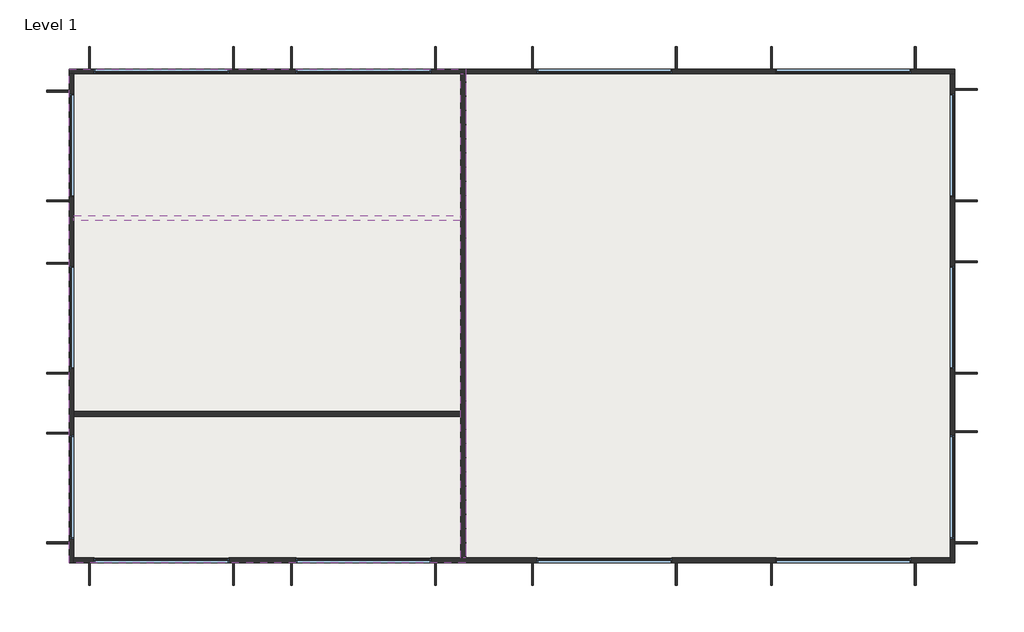
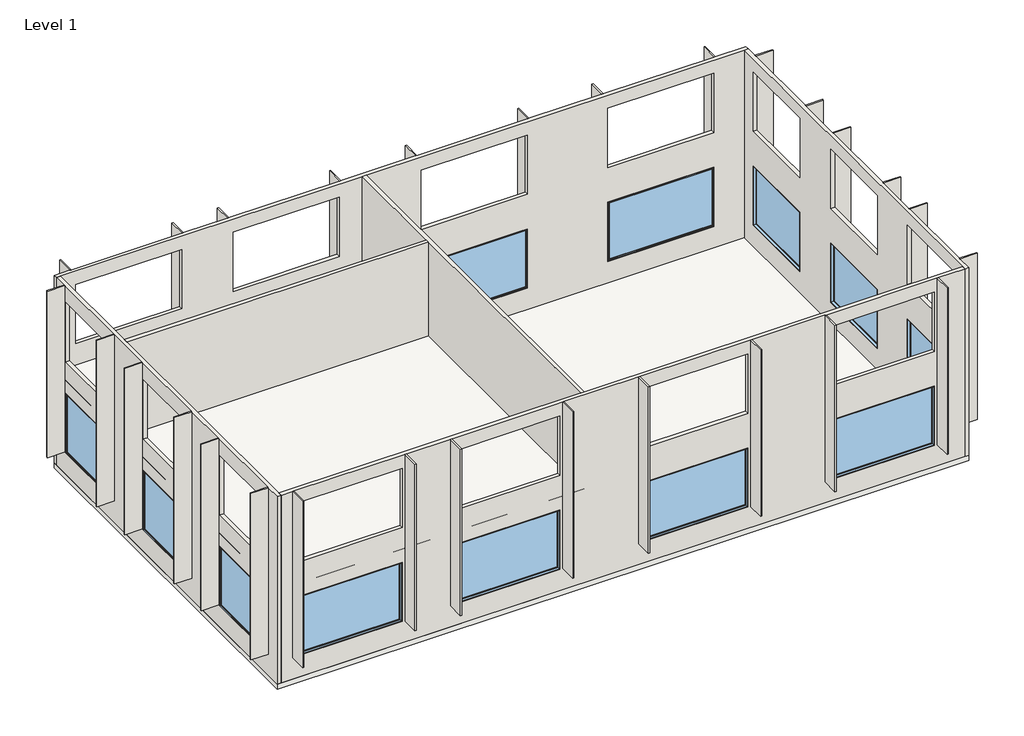
# One storey: 36 walls, 14 windows, 2 slabs.
"""IFC4 building model written with IfcOpenShell, lengths in millimetres."""

import ifcopenshell
import ifcopenshell.guid

model = None  # the IFC model being written
_history = None  # IfcOwnerHistory: only IFC2X3 demands one
_inside = {}  # id of a spatial element -> (the spatial element, [elements in it])
_under = {}  # id of a project, library or spatial element -> (it, [spatial elements below it])
_declared = {}  # id of a project -> (the project, [libraries it declares])
_typed = {}  # id of a type object -> (the type object, [elements of that type])
_made_of = {}  # id of a material, layer set ... -> (it, [elements and type objects made of it])


def new_model(schema):
    """Start an empty IFC model of exactly this schema.

    Asked for "IFC4X3", IfcOpenShell would pick the latest addendum, in which some entities
    have other attributes; the version numbers below select the first issue.
    IFC2X3 requires an IfcOwnerHistory on every rooted entity: one is made here for all.
    """
    global model, _history
    if schema == "IFC4X3":
        model = ifcopenshell.file(schema_version=(4, 3, 0, 0))
    else:
        model = ifcopenshell.file(schema=schema)
    _inside.clear()
    _under.clear()
    _declared.clear()
    _typed.clear()
    _made_of.clear()
    _history = None
    if model.schema == "IFC2X3":
        org = make("IfcOrganization", Name="unknown")
        user = make(
            "IfcPersonAndOrganization",
            ThePerson=make("IfcPerson", FamilyName="unknown"),
            TheOrganization=org,
        )
        app = make(
            "IfcApplication",
            ApplicationDeveloper=org,
            Version="unknown",
            ApplicationFullName="unknown",
            ApplicationIdentifier="unknown",
        )
        _history = make(
            "IfcOwnerHistory",
            OwningUser=user,
            OwningApplication=app,
            ChangeAction="ADDED",
            CreationDate=0,
        )
    return model


def make(cls, **values):
    """One entity of the class cls with the attributes given. An attribute that is None is left unset."""
    return model.create_entity(
        cls, **{name: value for name, value in values.items() if value is not None}
    )


def rooted(cls, **values):
    """An entity with a GlobalId (a new one), such as an element, a storey or a relation."""
    return make(cls, GlobalId=ifcopenshell.guid.new(), OwnerHistory=_history, **values)


def si_unit(unit_type, name, prefix=None):
    """IfcSIUnit, for example si_unit("LENGTHUNIT", "METRE", prefix="MILLI")."""
    return make("IfcSIUnit", UnitType=unit_type, Prefix=prefix, Name=name)


def assignment(units):
    """IfcUnitAssignment: the units of a project."""
    return None if units is None else make("IfcUnitAssignment", Units=units)


def point(xyz):
    """IfcCartesianPoint."""
    return None if xyz is None else make("IfcCartesianPoint", Coordinates=xyz)


def direction(xyz):
    """IfcDirection."""
    return None if xyz is None else make("IfcDirection", DirectionRatios=xyz)


def frame(location, z_axis=None, x_axis=None):
    """IfcAxis2Placement3D, a coordinate frame: its origin and axes. An axis left out is left unset."""
    return make(
        "IfcAxis2Placement3D",
        Location=point(location),
        Axis=direction(z_axis),
        RefDirection=direction(x_axis),
    )


def origin():
    """The frame at (0, 0, 0) with its axes left unset."""
    return frame((0.0, 0.0, 0.0))


def origin_with_axes():
    """The frame at (0, 0, 0) with the z axis (0, 0, 1) and the x axis (1, 0, 0) written out."""
    return frame((0.0, 0.0, 0.0), z_axis=(0.0, 0.0, 1.0), x_axis=(1.0, 0.0, 0.0))


def place(relative_to, where):
    """IfcLocalPlacement: puts the frame where relative to a parent placement (None: the world)."""
    return make(
        "IfcLocalPlacement", PlacementRelTo=relative_to, RelativePlacement=where
    )


def context(
    kind, dimensions, precision=None, world=None, true_north=None, identifier=None
):
    """IfcGeometricRepresentationContext, for example the 3D "Model" context."""
    return make(
        "IfcGeometricRepresentationContext",
        ContextIdentifier=identifier,
        ContextType=kind,
        CoordinateSpaceDimension=dimensions,
        Precision=precision,
        WorldCoordinateSystem=world,
        TrueNorth=true_north,
    )


def project(units=None, contexts=None):
    """IfcProject with its units and contexts."""
    return rooted(
        "IfcProject",
        Name="project",
        RepresentationContexts=contexts,
        UnitsInContext=assignment(units),
    )


def spatial(cls, under=None, at=None, **own):
    """A site, building, storey or space (cls), placed at a placement, below another one or the project."""
    s = rooted(cls, ObjectPlacement=at, **own)
    if under is not None:
        _under.setdefault(under.id(), (under, []))[1].append(s)
    return s


def polyline(points):
    """IfcPolyline through the points."""
    return make("IfcPolyline", Points=[point(p) for p in points])


def outline(outer, holes=None, kind="AREA"):
    """IfcArbitraryClosedProfileDef: a profile drawn as a closed curve; with holes, ...WithVoids."""
    if holes is None:
        return make("IfcArbitraryClosedProfileDef", ProfileType=kind, OuterCurve=outer)
    return make(
        "IfcArbitraryProfileDefWithVoids",
        ProfileType=kind,
        OuterCurve=outer,
        InnerCurves=holes,
    )


def extrude(swept, where, along, depth):
    """IfcExtrudedAreaSolid: the profile swept, set in the frame where, extruded along a direction by depth."""
    return make(
        "IfcExtrudedAreaSolid",
        SweptArea=swept,
        Position=where,
        ExtrudedDirection=direction(along),
        Depth=depth,
    )


def faces_of(points, faces, orient=None, outer=None):
    """IfcFace entities. A face is a list of loops; a loop is a list of indices into points, from 0.

    orient and outer hold one flag for each loop. By default every Orientation is true, the
    first loop of a face is its IfcFaceOuterBound and the others are IfcFaceBound.
    """
    made = []
    for i, loops in enumerate(faces):
        bounds = []
        for j, loop in enumerate(loops):
            is_outer = j == 0 if outer is None else outer[i][j]
            bounds.append(
                make(
                    "IfcFaceOuterBound" if is_outer else "IfcFaceBound",
                    Bound=make("IfcPolyLoop", Polygon=[points[k] for k in loop]),
                    Orientation=True if orient is None else orient[i][j],
                )
            )
        made.append(make("IfcFace", Bounds=bounds))
    return made


def faceted_brep(points, faces, orient=None, outer=None, voids=None):
    """IfcFacetedBrep: a solid bounded by flat faces; with voids (closed shells), ...WithVoids."""
    shared = [point(p) for p in points]
    hull = make("IfcClosedShell", CfsFaces=faces_of(shared, faces, orient, outer))
    if voids is None:
        return make("IfcFacetedBrep", Outer=hull)
    return make(
        "IfcFacetedBrepWithVoids",
        Outer=hull,
        Voids=[
            make(cls, CfsFaces=faces_of(shared, fs, o, b)) for cls, fs, o, b in voids
        ],
    )


def shape(context_of_items, identifier, shape_type, items):
    """IfcShapeRepresentation: the items that make up one representation, for example the "Body"."""
    return make(
        "IfcShapeRepresentation",
        ContextOfItems=context_of_items,
        RepresentationIdentifier=identifier,
        RepresentationType=shape_type,
        Items=items,
    )


def source(mapping_origin, context_of_items, identifier, shape_type, items):
    """IfcRepresentationMap: a shape defined once, which mapped items show again and again."""
    return make(
        "IfcRepresentationMap",
        MappingOrigin=mapping_origin,
        MappedRepresentation=shape(context_of_items, identifier, shape_type, items),
    )


def transform(
    local_origin,
    x_axis=None,
    y_axis=None,
    z_axis=None,
    scale=None,
    scale2=None,
    scale3=None,
    uniform=True,
):
    """IfcCartesianTransformationOperator3D, or its non-uniform kind. x_axis, y_axis, z_axis: its Axis1, 2, 3."""
    if uniform:
        return make(
            "IfcCartesianTransformationOperator3D",
            Axis1=direction(x_axis),
            Axis2=direction(y_axis),
            LocalOrigin=point(local_origin),
            Scale=scale,
            Axis3=direction(z_axis),
        )
    return make(
        "IfcCartesianTransformationOperator3DnonUniform",
        Axis1=direction(x_axis),
        Axis2=direction(y_axis),
        LocalOrigin=point(local_origin),
        Scale=scale,
        Axis3=direction(z_axis),
        Scale2=scale2,
        Scale3=scale3,
    )


def mapped(mapping_source, mapping_target):
    """IfcMappedItem: shows the shape of a source again, moved by a transform."""
    return make(
        "IfcMappedItem", MappingSource=mapping_source, MappingTarget=mapping_target
    )


def made_of(thing, what):
    """Note that an element or type object is made of a material, layer set ...; save() writes the relation."""
    if what is not None:
        _made_of.setdefault(what.id(), (what, []))[1].append(thing)
    return thing


def element(
    cls,
    number,
    at=None,
    inside=None,
    cuts=None,
    type_object=None,
    material=None,
    context=None,
    identifier="Body",
    shape_type=None,
    held_by="IfcProductDefinitionShape",
    body=None,
    shapes=None,
    **own,
):
    """One element of the class cls, such as IfcWall. Its Tag is "e" and its number.

    at: its placement. inside: the storey or other place that contains it. cuts: it is an
    opening in that element (IfcRelVoidsElement). A single representation is given by context,
    identifier, shape_type and body (its items); several are given by shapes. held_by: the class
    of the entity that holds the representations. save() writes the other relations.
    """
    e = rooted(cls, Tag="e%d" % number, ObjectPlacement=at, **own)
    if body is not None:
        shapes = [shape(context, identifier, shape_type, body)]
    if shapes is not None:
        e.Representation = make(held_by, Representations=shapes)
    if inside is not None:
        _inside.setdefault(inside.id(), (inside, []))[1].append(e)
    if cuts is not None:
        rooted(
            "IfcRelVoidsElement", RelatingBuildingElement=cuts, RelatedOpeningElement=e
        )
    if type_object is not None:
        _typed.setdefault(type_object.id(), (type_object, []))[1].append(e)
    return made_of(e, material)


def aggregate(whole, parts):
    """IfcRelAggregates: a whole, such as a stair, and the parts it consists of."""
    return rooted("IfcRelAggregates", RelatingObject=whole, RelatedObjects=parts)


def save(model, path):
    """Write the relations noted so far, then the file.

    IfcRelAggregates (storeys below a building ...), IfcRelContainedInSpatialStructure (elements
    in a storey), IfcRelDefinesByType, IfcRelAssociatesMaterial and IfcRelDeclares: one each for
    every whole, place, type object, material and project.
    """
    for whole, parts in _under.values():
        aggregate(whole, parts)
    for where, things in _inside.values():
        rooted(
            "IfcRelContainedInSpatialStructure",
            RelatedElements=things,
            RelatingStructure=where,
        )
    for kind, things in _typed.values():
        rooted("IfcRelDefinesByType", RelatedObjects=things, RelatingType=kind)
    for what, things in _made_of.values():
        rooted("IfcRelAssociatesMaterial", RelatedObjects=things, RelatingMaterial=what)
    for by, libraries in _declared.values():
        rooted("IfcRelDeclares", RelatingContext=by, RelatedDefinitions=libraries)
    model.write(path)


def m_fixed_2500x_4228mm_fd5e51e7(model_context):
    return source(origin(), model_context, "Body", "SweptSolid", [
        extrude(outline(polyline([(-2050.8, 54.2), (2050.8, 54.2), (2050.8, 42.2), (-2050.8, 42.2), (-2050.8, 54.2)])), frame((0.0, 0.0, 368.0), z_axis=(0.0, 0.0, 1.0), x_axis=(1.0, 0.0, 0.0)), (0.0, 0.0, 1.0), 2374.0),
        extrude(outline(polyline([(2786.0, -2094.8), (324.0, -2094.8), (324.0, 2094.8), (2786.0, 2094.8), (2786.0, -2094.8)]), holes=[polyline([(2742.0, -2050.8), (2742.0, 2050.8), (368.0, 2050.8), (368.0, -2050.8), (2742.0, -2050.8)])]), frame((0.0, 26.2, 0.0), z_axis=(0.0, 1.0, 0.0), x_axis=(0.0, 0.0, 1.0)), (0.0, 0.0, 1.0), 44.0),
        extrude(outline(polyline([(2805.0, -2113.8), (305.0, -2113.8), (305.0, 2113.8), (2805.0, 2113.8), (2805.0, -2113.8)]), holes=[polyline([(2786.0, -2094.8), (2786.0, 2094.8), (324.0, 2094.8), (324.0, -2094.8), (2786.0, -2094.8)])]), frame((0.0, 26.2, 0.0), z_axis=(0.0, 1.0, 0.0), x_axis=(0.0, 0.0, 1.0)), (0.0, 0.0, 1.0), 63.0),
        extrude(outline(polyline([(2805.0, -2113.8), (305.0, -2113.8), (305.0, 2113.8), (2805.0, 2113.8), (2805.0, -2113.8)]), holes=[polyline([(2773.0, -2081.8), (2773.0, 2081.8), (337.0, 2081.8), (337.0, -2081.8), (2773.0, -2081.8)])]), frame((0.0, -63.2, 0.0), z_axis=(0.0, 1.0, 0.0), x_axis=(0.0, 0.0, 1.0)), (0.0, 0.0, 1.0), 89.4),
    ])


def m_fixed_2500x_4228mm_f14c179f(model_context):
    return source(origin(), model_context, "Body", "SweptSolid", [
        extrude(outline(polyline([(-2050.8, -54.2), (-2050.8, -42.2), (2050.8, -42.2), (2050.8, -54.2), (-2050.8, -54.2)])), frame((0.0, 0.0, 368.0), z_axis=(0.0, 0.0, 1.0), x_axis=(1.0, 0.0, 0.0)), (0.0, 0.0, 1.0), 2374.0),
        extrude(outline(polyline([(2786.0, -2094.8), (324.0, -2094.8), (324.0, 2094.8), (2786.0, 2094.8), (2786.0, -2094.8)]), holes=[polyline([(2742.0, -2050.8), (2742.0, 2050.8), (368.0, 2050.8), (368.0, -2050.8), (2742.0, -2050.8)])]), frame((0.0, -70.2, 0.0), z_axis=(0.0, 1.0, 0.0), x_axis=(0.0, 0.0, 1.0)), (0.0, 0.0, 1.0), 44.0),
        extrude(outline(polyline([(2805.0, -2113.8), (305.0, -2113.8), (305.0, 2113.8), (2805.0, 2113.8), (2805.0, -2113.8)]), holes=[polyline([(2786.0, -2094.8), (2786.0, 2094.8), (324.0, 2094.8), (324.0, -2094.8), (2786.0, -2094.8)])]), frame((0.0, -89.2, 0.0), z_axis=(0.0, 1.0, 0.0), x_axis=(0.0, 0.0, 1.0)), (0.0, 0.0, 1.0), 63.0),
        extrude(outline(polyline([(2805.0, -2113.8), (305.0, -2113.8), (305.0, 2113.8), (2805.0, 2113.8), (2805.0, -2113.8)]), holes=[polyline([(2773.0, -2081.8), (2773.0, 2081.8), (337.0, 2081.8), (337.0, -2081.8), (2773.0, -2081.8)])]), frame((0.0, -26.2, 0.0), z_axis=(0.0, 1.0, 0.0), x_axis=(0.0, 0.0, 1.0)), (0.0, 0.0, 1.0), 89.4),
    ])


def m_fixed_2500x_3220mm_df94f4d0(model_context):
    return source(origin(), model_context, "Body", "SweptSolid", [
        extrude(outline(polyline([(-1546.8, 54.2), (1546.8, 54.2), (1546.8, 42.2), (-1546.8, 42.2), (-1546.8, 54.2)])), frame((0.0, 0.0, 368.0), z_axis=(0.0, 0.0, 1.0), x_axis=(1.0, 0.0, 0.0)), (0.0, 0.0, 1.0), 2374.0),
        extrude(outline(polyline([(2786.0, -1590.8), (324.0, -1590.8), (324.0, 1590.8), (2786.0, 1590.8), (2786.0, -1590.8)]), holes=[polyline([(2742.0, -1546.8), (2742.0, 1546.8), (368.0, 1546.8), (368.0, -1546.8), (2742.0, -1546.8)])]), frame((0.0, 26.2, 0.0), z_axis=(0.0, 1.0, 0.0), x_axis=(0.0, 0.0, 1.0)), (0.0, 0.0, 1.0), 44.0),
        extrude(outline(polyline([(2805.0, -1609.8), (305.0, -1609.8), (305.0, 1609.8), (2805.0, 1609.8), (2805.0, -1609.8)]), holes=[polyline([(2786.0, -1590.8), (2786.0, 1590.8), (324.0, 1590.8), (324.0, -1590.8), (2786.0, -1590.8)])]), frame((0.0, 26.2, 0.0), z_axis=(0.0, 1.0, 0.0), x_axis=(0.0, 0.0, 1.0)), (0.0, 0.0, 1.0), 63.0),
        extrude(outline(polyline([(2805.0, -1609.8), (305.0, -1609.8), (305.0, 1609.8), (2805.0, 1609.8), (2805.0, -1609.8)]), holes=[polyline([(2773.0, -1577.8), (2773.0, 1577.8), (337.0, 1577.8), (337.0, -1577.8), (2773.0, -1577.8)])]), frame((0.0, -63.2, 0.0), z_axis=(0.0, 1.0, 0.0), x_axis=(0.0, 0.0, 1.0)), (0.0, 0.0, 1.0), 89.4),
    ])


def m_fixed_2500x_3220mm_8b997f8c(model_context):
    return source(origin(), model_context, "Body", "SweptSolid", [
        extrude(outline(polyline([(-1546.8, -54.2), (-1546.8, -42.2), (1546.8, -42.2), (1546.8, -54.2), (-1546.8, -54.2)])), frame((0.0, 0.0, 368.0), z_axis=(0.0, 0.0, 1.0), x_axis=(1.0, 0.0, 0.0)), (0.0, 0.0, 1.0), 2374.0),
        extrude(outline(polyline([(2786.0, -1590.8), (324.0, -1590.8), (324.0, 1590.8), (2786.0, 1590.8), (2786.0, -1590.8)]), holes=[polyline([(2742.0, -1546.8), (2742.0, 1546.8), (368.0, 1546.8), (368.0, -1546.8), (2742.0, -1546.8)])]), frame((0.0, -70.2, 0.0), z_axis=(0.0, 1.0, 0.0), x_axis=(0.0, 0.0, 1.0)), (0.0, 0.0, 1.0), 44.0),
        extrude(outline(polyline([(2805.0, -1609.8), (305.0, -1609.8), (305.0, 1609.8), (2805.0, 1609.8), (2805.0, -1609.8)]), holes=[polyline([(2786.0, -1590.8), (2786.0, 1590.8), (324.0, 1590.8), (324.0, -1590.8), (2786.0, -1590.8)])]), frame((0.0, -89.2, 0.0), z_axis=(0.0, 1.0, 0.0), x_axis=(0.0, 0.0, 1.0)), (0.0, 0.0, 1.0), 63.0),
        extrude(outline(polyline([(2805.0, -1609.8), (305.0, -1609.8), (305.0, 1609.8), (2805.0, 1609.8), (2805.0, -1609.8)]), holes=[polyline([(2773.0, -1577.8), (2773.0, 1577.8), (337.0, 1577.8), (337.0, -1577.8), (2773.0, -1577.8)])]), frame((0.0, -26.2, 0.0), z_axis=(0.0, 1.0, 0.0), x_axis=(0.0, 0.0, 1.0)), (0.0, 0.0, 1.0), 89.4),
    ])


model = new_model("IFC4")

# Units and contexts
model_context = context("Model", 3, world=origin())
ifc_project = project(units=[si_unit("LENGTHUNIT", "METRE", prefix="MILLI")], contexts=[model_context])

# Site, building, storey
site = spatial("IfcSite", under=ifc_project)
building = spatial("IfcBuilding", under=site)
storey = spatial("IfcBuildingStorey", under=building, Name="Level 1", Elevation=0.0)

# Slabs
placement = place(None, origin())
element("IfcSlab", 1, ObjectType="160mm Concrete With 50mm Metal Deck", at=placement, inside=storey, context=model_context, shape_type="Brep", body=[
    faceted_brep([(29068.464681, 11296.9802217, -210.0), (29068.464681, -4095.4197783, -210.0), (1484.064681, -4095.4197783, -210.0), (1484.064681, 11296.9802217, -210.0), (29068.464681, 11296.9802217, 0.0), (1484.064681, 11296.9802217, 0.0), (1484.064681, -4095.4197783, 0.0), (28916.064681, -4095.4197783, 0.0), (29068.464681, -4095.4197783, 0.0), (29068.464681, 11144.5802217, 0.0)], [[[0, 1, 2, 3]], [[4, 5, 6, 7, 8, 9]], [[1, 0, 4, 9, 8]], [[2, 1, 8, 7, 6]], [[3, 2, 6, 5]], [[0, 3, 5, 4]]]),
])
element("IfcSlab", 2, ObjectType="160mm Concrete With 50mm Metal Deck", at=placement, inside=storey, context=model_context, shape_type="SweptSolid", body=[
    extrude(outline(polyline([(13828.464681, 11296.9802217), (13828.464681, -4095.4197783), (1484.064681, -4095.4197783), (1484.064681, 11296.9802217), (13828.464681, 11296.9802217)])), frame((0.0, 0.0, 3752.4), z_axis=(0.0, 0.0, 1.0), x_axis=(1.0, 0.0, 0.0)), (0.0, 0.0, 1.0), 210.0),
])

# Walls
element("IfcWall", 3, ObjectType="Generic - 152.4mm", at=placement, inside=storey, context=model_context, shape_type="Brep", body=[
    faceted_brep([(1484.064681, 11144.5802217, 0.0), (1636.464681, 11144.5802217, 0.0), (13676.064681, 11144.5802217, 0.0), (13828.464681, 11144.5802217, 0.0), (28916.064681, 11144.5802217, 0.0), (29068.464681, 11144.5802217, 0.0), (29068.464681, 11144.5802217, 7924.8), (28916.064681, 11144.5802217, 7924.8), (13828.464681, 11144.5802217, 7924.8), (13676.064681, 11144.5802217, 7924.8), (1636.464681, 11144.5802217, 7924.8), (1484.064681, 11144.5802217, 7924.8), (6474.064681, 11144.5802217, 902.4), (2246.464681, 11144.5802217, 902.4), (2246.464681, 11144.5802217, 3402.4), (6474.064681, 11144.5802217, 3402.4), (12766.064681, 11144.5802217, 902.4), (8538.464681, 11144.5802217, 902.4), (8538.464681, 11144.5802217, 3402.4), (12766.064681, 11144.5802217, 3402.4), (20266.064681, 11144.5802217, 902.4), (16038.464681, 11144.5802217, 902.4), (16038.464681, 11144.5802217, 3402.4), (20266.064681, 11144.5802217, 3402.4), (27706.064681, 11144.5802217, 902.4), (23478.464681, 11144.5802217, 902.4), (23478.464681, 11144.5802217, 3402.4), (27706.064681, 11144.5802217, 3402.4), (27706.064681, 11144.5802217, 4862.4), (23478.464681, 11144.5802217, 4862.4), (23478.464681, 11144.5802217, 7362.4), (27706.064681, 11144.5802217, 7362.4), (20266.064681, 11144.5802217, 4862.4), (16038.464681, 11144.5802217, 4862.4), (16038.464681, 11144.5802217, 7362.4), (20266.064681, 11144.5802217, 7362.4), (12766.064681, 11144.5802217, 4862.4), (8538.464681, 11144.5802217, 4862.4), (8538.464681, 11144.5802217, 7362.4), (12766.064681, 11144.5802217, 7362.4), (6474.064681, 11144.5802217, 4862.4), (2246.464681, 11144.5802217, 4862.4), (2246.464681, 11144.5802217, 7362.4), (6474.064681, 11144.5802217, 7362.4), (1484.064681, 11296.9802217, 0.0), (1484.064681, 11296.9802217, 7924.8), (2096.464681, 11296.9802217, 7924.8), (2146.464681, 11296.9802217, 7924.8), (6574.064681, 11296.9802217, 7924.8), (6624.064681, 11296.9802217, 7924.8), (8388.464681, 11296.9802217, 7924.8), (8438.464681, 11296.9802217, 7924.8), (12866.064681, 11296.9802217, 7924.8), (12916.064681, 11296.9802217, 7924.8), (15888.464681, 11296.9802217, 7924.8), (15938.464681, 11296.9802217, 7924.8), (20366.064681, 11296.9802217, 7924.8), (20416.064681, 11296.9802217, 7924.8), (23328.464681, 11296.9802217, 7924.8), (23378.464681, 11296.9802217, 7924.8), (27806.064681, 11296.9802217, 7924.8), (27856.064681, 11296.9802217, 7924.8), (29068.464681, 11296.9802217, 7924.8), (29068.464681, 11296.9802217, 0.0), (6474.064681, 11296.9802217, 902.4), (6474.064681, 11296.9802217, 3402.4), (2246.464681, 11296.9802217, 3402.4), (2246.464681, 11296.9802217, 902.4), (12766.064681, 11296.9802217, 902.4), (12766.064681, 11296.9802217, 3402.4), (8538.464681, 11296.9802217, 3402.4), (8538.464681, 11296.9802217, 902.4), (20266.064681, 11296.9802217, 902.4), (20266.064681, 11296.9802217, 3402.4), (16038.464681, 11296.9802217, 3402.4), (16038.464681, 11296.9802217, 902.4), (27706.064681, 11296.9802217, 902.4), (27706.064681, 11296.9802217, 3402.4), (23478.464681, 11296.9802217, 3402.4), (23478.464681, 11296.9802217, 902.4), (27706.064681, 11296.9802217, 4862.4), (27706.064681, 11296.9802217, 7362.4), (23478.464681, 11296.9802217, 7362.4), (23478.464681, 11296.9802217, 4862.4), (20266.064681, 11296.9802217, 4862.4), (20266.064681, 11296.9802217, 7362.4), (16038.464681, 11296.9802217, 7362.4), (16038.464681, 11296.9802217, 4862.4), (12766.064681, 11296.9802217, 4862.4), (12766.064681, 11296.9802217, 7362.4), (8538.464681, 11296.9802217, 7362.4), (8538.464681, 11296.9802217, 4862.4), (6474.064681, 11296.9802217, 4862.4), (6474.064681, 11296.9802217, 7362.4), (2246.464681, 11296.9802217, 7362.4), (2246.464681, 11296.9802217, 4862.4)], [[[0, 1, 2, 3, 4, 5, 6, 7, 8, 9, 10, 11], [12, 13, 14, 15], [16, 17, 18, 19], [20, 21, 22, 23], [24, 25, 26, 27], [28, 29, 30, 31], [32, 33, 34, 35], [36, 37, 38, 39], [40, 41, 42, 43]], [[44, 45, 46, 47, 48, 49, 50, 51, 52, 53, 54, 55, 56, 57, 58, 59, 60, 61, 62, 63], [64, 65, 66, 67], [68, 69, 70, 71], [72, 73, 74, 75], [76, 77, 78, 79], [80, 81, 82, 83], [84, 85, 86, 87], [88, 89, 90, 91], [92, 93, 94, 95]], [[5, 4, 3, 2, 1, 0, 44, 63]], [[11, 10, 9, 8, 7, 6, 62, 61, 60, 59, 58, 57, 56, 55, 54, 53, 52, 51, 50, 49, 48, 47, 46, 45]], [[6, 5, 63, 62]], [[0, 11, 45, 44]], [[65, 64, 12, 15]], [[66, 65, 15, 14]], [[67, 66, 14, 13]], [[64, 67, 13, 12]], [[69, 68, 16, 19]], [[70, 69, 19, 18]], [[71, 70, 18, 17]], [[68, 71, 17, 16]], [[73, 72, 20, 23]], [[74, 73, 23, 22]], [[75, 74, 22, 21]], [[72, 75, 21, 20]], [[77, 76, 24, 27]], [[78, 77, 27, 26]], [[79, 78, 26, 25]], [[76, 79, 25, 24]], [[81, 80, 28, 31]], [[82, 81, 31, 30]], [[83, 82, 30, 29]], [[80, 83, 29, 28]], [[85, 84, 32, 35]], [[86, 85, 35, 34]], [[87, 86, 34, 33]], [[84, 87, 33, 32]], [[89, 88, 36, 39]], [[90, 89, 39, 38]], [[91, 90, 38, 37]], [[88, 91, 37, 36]], [[93, 92, 40, 43]], [[94, 93, 43, 42]], [[95, 94, 42, 41]], [[92, 95, 41, 40]]]),
])
element("IfcWall", 4, ObjectType="Generic - 152.4mm", at=placement, inside=storey, context=model_context, shape_type="Brep", body=[
    faceted_brep([(28916.064681, 11144.5802217, 0.0), (28916.064681, -3943.0197783, 0.0), (28916.064681, -4095.4197783, 0.0), (28916.064681, -4095.4197783, 7924.8), (28916.064681, -3943.0197783, 7924.8), (28916.064681, 11144.5802217, 7924.8), (28916.064681, -3343.0197783, 902.4), (28916.064681, -123.4197783, 902.4), (28916.064681, -123.4197783, 3402.4), (28916.064681, -3343.0197783, 3402.4), (28916.064681, 1942.9802217, 902.4), (28916.064681, 5162.5802217, 902.4), (28916.064681, 5162.5802217, 3402.4), (28916.064681, 1942.9802217, 3402.4), (28916.064681, 7310.9802217, 902.4), (28916.064681, 10530.5802217, 902.4), (28916.064681, 10530.5802217, 3402.4), (28916.064681, 7310.9802217, 3402.4), (28916.064681, -3343.0197783, 4864.8), (28916.064681, -123.4197783, 4864.8), (28916.064681, -123.4197783, 7364.8), (28916.064681, -3343.0197783, 7364.8), (28916.064681, 1942.9802217, 4864.8), (28916.064681, 5162.5802217, 4864.8), (28916.064681, 5162.5802217, 7364.8), (28916.064681, 1942.9802217, 7364.8), (28916.064681, 7310.9802217, 4864.8), (28916.064681, 10530.5802217, 4864.8), (28916.064681, 10530.5802217, 7364.8), (28916.064681, 7310.9802217, 7364.8), (29068.464681, 11144.5802217, 0.0), (29068.464681, 11144.5802217, 7924.8), (29068.464681, 10680.5802217, 7924.8), (29068.464681, 10630.5802217, 7924.8), (29068.464681, 7210.9802217, 7924.8), (29068.464681, 7160.9802217, 7924.8), (29068.464681, 5312.5802217, 7924.8), (29068.464681, 5262.5802217, 7924.8), (29068.464681, 1842.9802217, 7924.8), (29068.464681, 1792.9802217, 7924.8), (29068.464681, 26.5802217, 7924.8), (29068.464681, -23.4197783, 7924.8), (29068.464681, -3443.0197783, 7924.8), (29068.464681, -3493.0197783, 7924.8), (29068.464681, -4095.4197783, 7924.8), (29068.464681, -4095.4197783, 0.0), (29068.464681, -3343.0197783, 902.4), (29068.464681, -3343.0197783, 3402.4), (29068.464681, -123.4197783, 3402.4), (29068.464681, -123.4197783, 902.4), (29068.464681, 1942.9802217, 902.4), (29068.464681, 1942.9802217, 3402.4), (29068.464681, 5162.5802217, 3402.4), (29068.464681, 5162.5802217, 902.4), (29068.464681, 7310.9802217, 902.4), (29068.464681, 7310.9802217, 3402.4), (29068.464681, 10530.5802217, 3402.4), (29068.464681, 10530.5802217, 902.4), (29068.464681, -3343.0197783, 4864.8), (29068.464681, -3343.0197783, 7364.8), (29068.464681, -123.4197783, 7364.8), (29068.464681, -123.4197783, 4864.8), (29068.464681, 1942.9802217, 4864.8), (29068.464681, 1942.9802217, 7364.8), (29068.464681, 5162.5802217, 7364.8), (29068.464681, 5162.5802217, 4864.8), (29068.464681, 7310.9802217, 4864.8), (29068.464681, 7310.9802217, 7364.8), (29068.464681, 10530.5802217, 7364.8), (29068.464681, 10530.5802217, 4864.8)], [[[0, 1, 2, 3, 4, 5], [6, 7, 8, 9], [10, 11, 12, 13], [14, 15, 16, 17], [18, 19, 20, 21], [22, 23, 24, 25], [26, 27, 28, 29]], [[30, 31, 32, 33, 34, 35, 36, 37, 38, 39, 40, 41, 42, 43, 44, 45], [46, 47, 48, 49], [50, 51, 52, 53], [54, 55, 56, 57], [58, 59, 60, 61], [62, 63, 64, 65], [66, 67, 68, 69]], [[2, 1, 0, 30, 45]], [[5, 4, 3, 44, 43, 42, 41, 40, 39, 38, 37, 36, 35, 34, 33, 32, 31]], [[0, 5, 31, 30]], [[47, 46, 6, 9]], [[48, 47, 9, 8]], [[49, 48, 8, 7]], [[46, 49, 7, 6]], [[51, 50, 10, 13]], [[52, 51, 13, 12]], [[53, 52, 12, 11]], [[50, 53, 11, 10]], [[55, 54, 14, 17]], [[56, 55, 17, 16]], [[57, 56, 16, 15]], [[54, 57, 15, 14]], [[3, 2, 45, 44]], [[59, 58, 18, 21]], [[60, 59, 21, 20]], [[61, 60, 20, 19]], [[58, 61, 19, 18]], [[63, 62, 22, 25]], [[64, 63, 25, 24]], [[65, 64, 24, 23]], [[62, 65, 23, 22]], [[67, 66, 26, 29]], [[68, 67, 29, 28]], [[69, 68, 28, 27]], [[66, 69, 27, 26]]]),
])
element("IfcWall", 5, ObjectType="Generic - 152.4mm", at=placement, inside=storey, context=model_context, shape_type="Brep", body=[
    faceted_brep([(28916.064681, -3943.0197783, 0.0), (13828.464681, -3943.0197783, 0.0), (13676.064681, -3943.0197783, 0.0), (1636.464681, -3943.0197783, 0.0), (1636.464681, -3943.0197783, 7924.8), (13676.064681, -3943.0197783, 7924.8), (13828.464681, -3943.0197783, 7924.8), (28916.064681, -3943.0197783, 7924.8), (27706.064681, -3943.0197783, 902.4), (27706.064681, -3943.0197783, 3402.4), (23478.464681, -3943.0197783, 3402.4), (23478.464681, -3943.0197783, 902.4), (20266.064681, -3943.0197783, 902.4), (20266.064681, -3943.0197783, 3402.4), (16038.464681, -3943.0197783, 3402.4), (16038.464681, -3943.0197783, 902.4), (12766.064681, -3943.0197783, 902.4), (12766.064681, -3943.0197783, 3402.4), (8538.464681, -3943.0197783, 3402.4), (8538.464681, -3943.0197783, 902.4), (6474.064681, -3943.0197783, 902.4), (6474.064681, -3943.0197783, 3402.4), (2246.464681, -3943.0197783, 3402.4), (2246.464681, -3943.0197783, 902.4), (27706.064681, -3943.0197783, 4862.4), (27706.064681, -3943.0197783, 7362.4), (23478.464681, -3943.0197783, 7362.4), (23478.464681, -3943.0197783, 4862.4), (20266.064681, -3943.0197783, 4862.4), (20266.064681, -3943.0197783, 7362.4), (16038.464681, -3943.0197783, 7362.4), (16038.464681, -3943.0197783, 4862.4), (12766.064681, -3943.0197783, 4862.4), (12766.064681, -3943.0197783, 7362.4), (8538.464681, -3943.0197783, 7362.4), (8538.464681, -3943.0197783, 4862.4), (6474.064681, -3943.0197783, 4862.4), (6474.064681, -3943.0197783, 7362.4), (2246.464681, -3943.0197783, 7362.4), (2246.464681, -3943.0197783, 4862.4), (28916.064681, -4095.4197783, 0.0), (28916.064681, -4095.4197783, 7924.8), (27856.064681, -4095.4197783, 7924.8), (27806.064681, -4095.4197783, 7924.8), (23378.464681, -4095.4197783, 7924.8), (23328.464681, -4095.4197783, 7924.8), (20416.064681, -4095.4197783, 7924.8), (20366.064681, -4095.4197783, 7924.8), (15938.464681, -4095.4197783, 7924.8), (15888.464681, -4095.4197783, 7924.8), (12916.064681, -4095.4197783, 7924.8), (12866.064681, -4095.4197783, 7924.8), (8438.464681, -4095.4197783, 7924.8), (8388.464681, -4095.4197783, 7924.8), (6624.064681, -4095.4197783, 7924.8), (6574.064681, -4095.4197783, 7924.8), (2146.464681, -4095.4197783, 7924.8), (2096.464681, -4095.4197783, 7924.8), (1636.464681, -4095.4197783, 7924.8), (1636.464681, -4095.4197783, 0.0), (27706.064681, -4095.4197783, 902.4), (23478.464681, -4095.4197783, 902.4), (23478.464681, -4095.4197783, 3402.4), (27706.064681, -4095.4197783, 3402.4), (20266.064681, -4095.4197783, 902.4), (16038.464681, -4095.4197783, 902.4), (16038.464681, -4095.4197783, 3402.4), (20266.064681, -4095.4197783, 3402.4), (12766.064681, -4095.4197783, 902.4), (8538.464681, -4095.4197783, 902.4), (8538.464681, -4095.4197783, 3402.4), (12766.064681, -4095.4197783, 3402.4), (6474.064681, -4095.4197783, 902.4), (2246.464681, -4095.4197783, 902.4), (2246.464681, -4095.4197783, 3402.4), (6474.064681, -4095.4197783, 3402.4), (27706.064681, -4095.4197783, 4862.4), (23478.464681, -4095.4197783, 4862.4), (23478.464681, -4095.4197783, 7362.4), (27706.064681, -4095.4197783, 7362.4), (20266.064681, -4095.4197783, 4862.4), (16038.464681, -4095.4197783, 4862.4), (16038.464681, -4095.4197783, 7362.4), (20266.064681, -4095.4197783, 7362.4), (12766.064681, -4095.4197783, 4862.4), (8538.464681, -4095.4197783, 4862.4), (8538.464681, -4095.4197783, 7362.4), (12766.064681, -4095.4197783, 7362.4), (6474.064681, -4095.4197783, 4862.4), (2246.464681, -4095.4197783, 4862.4), (2246.464681, -4095.4197783, 7362.4), (6474.064681, -4095.4197783, 7362.4)], [[[0, 1, 2, 3, 4, 5, 6, 7], [8, 9, 10, 11], [12, 13, 14, 15], [16, 17, 18, 19], [20, 21, 22, 23], [24, 25, 26, 27], [28, 29, 30, 31], [32, 33, 34, 35], [36, 37, 38, 39]], [[40, 41, 42, 43, 44, 45, 46, 47, 48, 49, 50, 51, 52, 53, 54, 55, 56, 57, 58, 59], [60, 61, 62, 63], [64, 65, 66, 67], [68, 69, 70, 71], [72, 73, 74, 75], [76, 77, 78, 79], [80, 81, 82, 83], [84, 85, 86, 87], [88, 89, 90, 91]], [[3, 2, 1, 0, 40, 59]], [[7, 6, 5, 4, 58, 57, 56, 55, 54, 53, 52, 51, 50, 49, 48, 47, 46, 45, 44, 43, 42, 41]], [[9, 8, 60, 63]], [[10, 9, 63, 62]], [[11, 10, 62, 61]], [[8, 11, 61, 60]], [[13, 12, 64, 67]], [[14, 13, 67, 66]], [[15, 14, 66, 65]], [[12, 15, 65, 64]], [[17, 16, 68, 71]], [[18, 17, 71, 70]], [[19, 18, 70, 69]], [[16, 19, 69, 68]], [[21, 20, 72, 75]], [[22, 21, 75, 74]], [[23, 22, 74, 73]], [[20, 23, 73, 72]], [[0, 7, 41, 40]], [[4, 3, 59, 58]], [[25, 24, 76, 79]], [[26, 25, 79, 78]], [[27, 26, 78, 77]], [[24, 27, 77, 76]], [[29, 28, 80, 83]], [[30, 29, 83, 82]], [[31, 30, 82, 81]], [[28, 31, 81, 80]], [[33, 32, 84, 87]], [[34, 33, 87, 86]], [[35, 34, 86, 85]], [[32, 35, 85, 84]], [[37, 36, 88, 91]], [[38, 37, 91, 90]], [[39, 38, 90, 89]], [[36, 39, 89, 88]]]),
])
element("IfcWall", 6, ObjectType="Generic - 152.4mm", at=placement, inside=storey, context=model_context, shape_type="Brep", body=[
    faceted_brep([(1636.464681, -4095.4197783, 0.0), (1636.464681, -3943.0197783, 0.0), (1636.464681, 476.5802217, 0.0), (1636.464681, 628.9802217, 0.0), (1636.464681, 11144.5802217, 0.0), (1636.464681, 11144.5802217, 7924.8), (1636.464681, 6724.9802217, 7924.8), (1636.464681, 6572.5802217, 7924.8), (1636.464681, -3943.0197783, 7924.8), (1636.464681, -4095.4197783, 7924.8), (1636.464681, 7310.9802217, 4734.5029682), (1636.464681, 7310.9802217, 7234.5029682), (1636.464681, 10530.5802217, 7234.5029682), (1636.464681, 10530.5802217, 4734.5029682), (1636.464681, 1942.9802217, 4734.5029682), (1636.464681, 1942.9802217, 7234.5029682), (1636.464681, 5162.5802217, 7234.5029682), (1636.464681, 5162.5802217, 4734.5029682), (1636.464681, -3343.0197783, 4734.5029682), (1636.464681, -3343.0197783, 7234.5029682), (1636.464681, -123.4197783, 7234.5029682), (1636.464681, -123.4197783, 4734.5029682), (1636.464681, -3343.0197783, 902.4), (1636.464681, -3343.0197783, 3402.4), (1636.464681, -123.4197783, 3402.4), (1636.464681, -123.4197783, 902.4), (1636.464681, 7310.9802217, 902.4), (1636.464681, 7310.9802217, 3402.4), (1636.464681, 10530.5802217, 3402.4), (1636.464681, 10530.5802217, 902.4), (1636.464681, 1942.9802217, 902.4), (1636.464681, 1942.9802217, 3402.4), (1636.464681, 5162.5802217, 3402.4), (1636.464681, 5162.5802217, 902.4), (1484.064681, -4095.4197783, 0.0), (1484.064681, -4095.4197783, 7924.8), (1484.064681, -3493.0197783, 7924.8), (1484.064681, -3443.0197783, 7924.8), (1484.064681, -73.4197783, 7924.8), (1484.064681, -23.4197783, 7924.8), (1484.064681, 1792.9802217, 7924.8), (1484.064681, 1842.9802217, 7924.8), (1484.064681, 5212.5802217, 7924.8), (1484.064681, 5262.5802217, 7924.8), (1484.064681, 7160.9802217, 7924.8), (1484.064681, 7210.9802217, 7924.8), (1484.064681, 10580.5802217, 7924.8), (1484.064681, 10630.5802217, 7924.8), (1484.064681, 11144.5802217, 7924.8), (1484.064681, 11144.5802217, 0.0), (1484.064681, 7310.9802217, 4734.5029682), (1484.064681, 10530.5802217, 4734.5029682), (1484.064681, 10530.5802217, 7234.5029682), (1484.064681, 7310.9802217, 7234.5029682), (1484.064681, 1942.9802217, 4734.5029682), (1484.064681, 5162.5802217, 4734.5029682), (1484.064681, 5162.5802217, 7234.5029682), (1484.064681, 1942.9802217, 7234.5029682), (1484.064681, -3343.0197783, 4734.5029682), (1484.064681, -123.4197783, 4734.5029682), (1484.064681, -123.4197783, 7234.5029682), (1484.064681, -3343.0197783, 7234.5029682), (1484.064681, -3343.0197783, 902.4), (1484.064681, -123.4197783, 902.4), (1484.064681, -123.4197783, 3402.4), (1484.064681, -3343.0197783, 3402.4), (1484.064681, 7310.9802217, 902.4), (1484.064681, 10530.5802217, 902.4), (1484.064681, 10530.5802217, 3402.4), (1484.064681, 7310.9802217, 3402.4), (1484.064681, 1942.9802217, 902.4), (1484.064681, 5162.5802217, 902.4), (1484.064681, 5162.5802217, 3402.4), (1484.064681, 1942.9802217, 3402.4)], [[[0, 1, 2, 3, 4, 5, 6, 7, 8, 9], [10, 11, 12, 13], [14, 15, 16, 17], [18, 19, 20, 21], [22, 23, 24, 25], [26, 27, 28, 29], [30, 31, 32, 33]], [[34, 35, 36, 37, 38, 39, 40, 41, 42, 43, 44, 45, 46, 47, 48, 49], [50, 51, 52, 53], [54, 55, 56, 57], [58, 59, 60, 61], [62, 63, 64, 65], [66, 67, 68, 69], [70, 71, 72, 73]], [[4, 3, 2, 1, 0, 34, 49]], [[9, 8, 7, 6, 5, 48, 47, 46, 45, 44, 43, 42, 41, 40, 39, 38, 37, 36, 35]], [[5, 4, 49, 48]], [[0, 9, 35, 34]], [[11, 10, 50, 53]], [[12, 11, 53, 52]], [[13, 12, 52, 51]], [[10, 13, 51, 50]], [[15, 14, 54, 57]], [[16, 15, 57, 56]], [[17, 16, 56, 55]], [[14, 17, 55, 54]], [[19, 18, 58, 61]], [[20, 19, 61, 60]], [[21, 20, 60, 59]], [[18, 21, 59, 58]], [[23, 22, 62, 65]], [[24, 23, 65, 64]], [[25, 24, 64, 63]], [[22, 25, 63, 62]], [[27, 26, 66, 69]], [[28, 27, 69, 68]], [[29, 28, 68, 67]], [[26, 29, 67, 66]], [[31, 30, 70, 73]], [[32, 31, 73, 72]], [[33, 32, 72, 71]], [[30, 33, 71, 70]]]),
])
element("IfcWall", 7, ObjectType="Generic - 152.4mm - Interior", at=placement, inside=storey, context=model_context, shape_type="Brep", body=[
    faceted_brep([(13828.464681, -3943.0197783, 0.0), (13828.464681, 11144.5802217, 0.0), (13828.464681, 11144.5802217, 3752.4), (13828.464681, -3943.0197783, 3752.4), (13676.064681, -3943.0197783, 0.0), (13676.064681, -3943.0197783, 3752.4), (13676.064681, 476.5802217, 3752.4), (13676.064681, 628.9802217, 3752.4), (13676.064681, 11144.5802217, 3752.4), (13676.064681, 11144.5802217, 0.0), (13676.064681, 628.9802217, 0.0), (13676.064681, 476.5802217, 0.0)], [[[0, 1, 2, 3]], [[4, 5, 6, 7, 8, 9, 10, 11]], [[1, 0, 4, 11, 10, 9]], [[0, 3, 5, 4]], [[2, 1, 9, 8]], [[3, 2, 8, 7, 6, 5]]]),
])
element("IfcWall", 8, ObjectType="Generic - 152.4mm - Interior", at=placement, inside=storey, context=model_context, shape_type="SweptSolid", body=[
    extrude(outline(polyline([(1636.464681, 628.9802217), (13676.064681, 628.9802217), (13676.064681, 476.5802217), (1636.464681, 476.5802217), (1636.464681, 628.9802217)])), origin_with_axes(), (0.0, 0.0, 1.0), 3752.4),
])
element("IfcWall", 9, ObjectType="Generic - 152.4mm - Interior", at=placement, inside=storey, context=model_context, shape_type="Brep", body=[
    faceted_brep([(13676.064681, 11144.5802217, 3962.4), (13676.064681, 6724.9802217, 3962.4), (13676.064681, 6572.5802217, 3962.4), (13676.064681, -3943.0197783, 3962.4), (13676.064681, -3943.0197783, 7924.8), (13676.064681, 6572.5802217, 7924.8), (13676.064681, 6724.9802217, 7924.8), (13676.064681, 11144.5802217, 7924.8), (13828.464681, 11144.5802217, 3962.4), (13828.464681, 11144.5802217, 7924.8), (13828.464681, -3943.0197783, 7924.8), (13828.464681, -3943.0197783, 3962.4)], [[[0, 1, 2, 3, 4, 5, 6, 7]], [[8, 9, 10, 11]], [[3, 2, 1, 0, 8, 11]], [[7, 6, 5, 4, 10, 9]], [[4, 3, 11, 10]], [[0, 7, 9, 8]]]),
])
element("IfcWall", 10, ObjectType="Generic - 152.4mm - Interior", at=placement, inside=storey, context=model_context, shape_type="SweptSolid", body=[
    extrude(outline(polyline([(1636.464681, 6724.9802217), (13676.064681, 6724.9802217), (13676.064681, 6572.5802217), (1636.464681, 6572.5802217), (1636.464681, 6724.9802217)])), frame((0.0, 0.0, 3962.4), z_axis=(0.0, 0.0, 1.0), x_axis=(1.0, 0.0, 0.0)), (0.0, 0.0, 1.0), 3962.4),
])
element("IfcWall", 11, ObjectType="Shading devices", at=placement, inside=storey, context=model_context, shape_type="SweptSolid", body=[
    extrude(outline(polyline([(2096.464681, -4795.4197783), (2096.464681, -4095.4197783), (2146.464681, -4095.4197783), (2146.464681, -4795.4197783), (2096.464681, -4795.4197783)])), frame((0.0, 0.0, 902.4), z_axis=(0.0, 0.0, 1.0), x_axis=(1.0, 0.0, 0.0)), (0.0, 0.0, 1.0), 7022.4),
])
element("IfcWall", 12, ObjectType="Shading devices", at=placement, inside=storey, context=model_context, shape_type="SweptSolid", body=[
    extrude(outline(polyline([(6574.064681, -4795.4197783), (6574.064681, -4095.4197783), (6624.064681, -4095.4197783), (6624.064681, -4795.4197783), (6574.064681, -4795.4197783)])), frame((0.0, 0.0, 902.4), z_axis=(0.0, 0.0, 1.0), x_axis=(1.0, 0.0, 0.0)), (0.0, 0.0, 1.0), 7022.4),
])
element("IfcWall", 13, ObjectType="Shading devices", at=placement, inside=storey, context=model_context, shape_type="SweptSolid", body=[
    extrude(outline(polyline([(8388.464681, -4795.4197783), (8388.464681, -4095.4197783), (8438.464681, -4095.4197783), (8438.464681, -4795.4197783), (8388.464681, -4795.4197783)])), frame((0.0, 0.0, 902.4), z_axis=(0.0, 0.0, 1.0), x_axis=(1.0, 0.0, 0.0)), (0.0, 0.0, 1.0), 7022.4),
])
element("IfcWall", 14, ObjectType="Shading devices", at=placement, inside=storey, context=model_context, shape_type="SweptSolid", body=[
    extrude(outline(polyline([(12866.064681, -4795.4197783), (12866.064681, -4095.4197783), (12916.064681, -4095.4197783), (12916.064681, -4795.4197783), (12866.064681, -4795.4197783)])), frame((0.0, 0.0, 902.4), z_axis=(0.0, 0.0, 1.0), x_axis=(1.0, 0.0, 0.0)), (0.0, 0.0, 1.0), 7022.4),
])
element("IfcWall", 15, ObjectType="Shading devices", at=placement, inside=storey, context=model_context, shape_type="SweptSolid", body=[
    extrude(outline(polyline([(15888.464681, -4795.4197783), (15888.464681, -4095.4197783), (15938.464681, -4095.4197783), (15938.464681, -4795.4197783), (15888.464681, -4795.4197783)])), frame((0.0, 0.0, 902.4), z_axis=(0.0, 0.0, 1.0), x_axis=(1.0, 0.0, 0.0)), (0.0, 0.0, 1.0), 7022.4),
])
element("IfcWall", 16, ObjectType="Shading devices", at=placement, inside=storey, context=model_context, shape_type="SweptSolid", body=[
    extrude(outline(polyline([(20366.064681, -4795.4197783), (20366.064681, -4095.4197783), (20416.064681, -4095.4197783), (20416.064681, -4795.4197783), (20366.064681, -4795.4197783)])), frame((0.0, 0.0, 902.4), z_axis=(0.0, 0.0, 1.0), x_axis=(1.0, 0.0, 0.0)), (0.0, 0.0, 1.0), 7022.4),
])
element("IfcWall", 17, ObjectType="Shading devices", at=placement, inside=storey, context=model_context, shape_type="SweptSolid", body=[
    extrude(outline(polyline([(23328.464681, -4795.4197783), (23328.464681, -4095.4197783), (23378.464681, -4095.4197783), (23378.464681, -4795.4197783), (23328.464681, -4795.4197783)])), frame((0.0, 0.0, 902.4), z_axis=(0.0, 0.0, 1.0), x_axis=(1.0, 0.0, 0.0)), (0.0, 0.0, 1.0), 7022.4),
])
element("IfcWall", 18, ObjectType="Shading devices", at=placement, inside=storey, context=model_context, shape_type="SweptSolid", body=[
    extrude(outline(polyline([(27806.064681, -4795.4197783), (27806.064681, -4095.4197783), (27856.064681, -4095.4197783), (27856.064681, -4795.4197783), (27806.064681, -4795.4197783)])), frame((0.0, 0.0, 902.4), z_axis=(0.0, 0.0, 1.0), x_axis=(1.0, 0.0, 0.0)), (0.0, 0.0, 1.0), 7022.4),
])
element("IfcWall", 19, ObjectType="Shading devices", at=placement, inside=storey, context=model_context, shape_type="SweptSolid", body=[
    extrude(outline(polyline([(29768.464681, 7160.9802217), (29068.464681, 7160.9802217), (29068.464681, 7210.9802217), (29768.464681, 7210.9802217), (29768.464681, 7160.9802217)])), frame((0.0, 0.0, 902.4), z_axis=(0.0, 0.0, 1.0), x_axis=(1.0, 0.0, 0.0)), (0.0, 0.0, 1.0), 7022.4),
])
element("IfcWall", 20, ObjectType="Shading devices", at=placement, inside=storey, context=model_context, shape_type="SweptSolid", body=[
    extrude(outline(polyline([(29768.464681, 10630.5802217), (29068.464681, 10630.5802217), (29068.464681, 10680.5802217), (29768.464681, 10680.5802217), (29768.464681, 10630.5802217)])), frame((0.0, 0.0, 902.4), z_axis=(0.0, 0.0, 1.0), x_axis=(1.0, 0.0, 0.0)), (0.0, 0.0, 1.0), 7022.4),
])
element("IfcWall", 21, ObjectType="Shading devices", at=placement, inside=storey, context=model_context, shape_type="SweptSolid", body=[
    extrude(outline(polyline([(27856.064681, 11996.9802217), (27856.064681, 11296.9802217), (27806.064681, 11296.9802217), (27806.064681, 11996.9802217), (27856.064681, 11996.9802217)])), frame((0.0, 0.0, 902.4), z_axis=(0.0, 0.0, 1.0), x_axis=(1.0, 0.0, 0.0)), (0.0, 0.0, 1.0), 7022.4),
])
element("IfcWall", 22, ObjectType="Shading devices", at=placement, inside=storey, context=model_context, shape_type="SweptSolid", body=[
    extrude(outline(polyline([(23378.464681, 11996.9802217), (23378.464681, 11296.9802217), (23328.464681, 11296.9802217), (23328.464681, 11996.9802217), (23378.464681, 11996.9802217)])), frame((0.0, 0.0, 902.4), z_axis=(0.0, 0.0, 1.0), x_axis=(1.0, 0.0, 0.0)), (0.0, 0.0, 1.0), 7022.4),
])
element("IfcWall", 23, ObjectType="Shading devices", at=placement, inside=storey, context=model_context, shape_type="SweptSolid", body=[
    extrude(outline(polyline([(20416.064681, 11996.9802217), (20416.064681, 11296.9802217), (20366.064681, 11296.9802217), (20366.064681, 11996.9802217), (20416.064681, 11996.9802217)])), frame((0.0, 0.0, 902.4), z_axis=(0.0, 0.0, 1.0), x_axis=(1.0, 0.0, 0.0)), (0.0, 0.0, 1.0), 7022.4),
])
element("IfcWall", 24, ObjectType="Shading devices", at=placement, inside=storey, context=model_context, shape_type="SweptSolid", body=[
    extrude(outline(polyline([(15938.464681, 11996.9802217), (15938.464681, 11296.9802217), (15888.464681, 11296.9802217), (15888.464681, 11996.9802217), (15938.464681, 11996.9802217)])), frame((0.0, 0.0, 902.4), z_axis=(0.0, 0.0, 1.0), x_axis=(1.0, 0.0, 0.0)), (0.0, 0.0, 1.0), 7022.4),
])
element("IfcWall", 25, ObjectType="Shading devices", at=placement, inside=storey, context=model_context, shape_type="SweptSolid", body=[
    extrude(outline(polyline([(12916.064681, 11996.9802217), (12916.064681, 11296.9802217), (12866.064681, 11296.9802217), (12866.064681, 11996.9802217), (12916.064681, 11996.9802217)])), frame((0.0, 0.0, 902.4), z_axis=(0.0, 0.0, 1.0), x_axis=(1.0, 0.0, 0.0)), (0.0, 0.0, 1.0), 7022.4),
])
element("IfcWall", 26, ObjectType="Shading devices", at=placement, inside=storey, context=model_context, shape_type="SweptSolid", body=[
    extrude(outline(polyline([(8438.464681, 11996.9802217), (8438.464681, 11296.9802217), (8388.464681, 11296.9802217), (8388.464681, 11996.9802217), (8438.464681, 11996.9802217)])), frame((0.0, 0.0, 902.4), z_axis=(0.0, 0.0, 1.0), x_axis=(1.0, 0.0, 0.0)), (0.0, 0.0, 1.0), 7022.4),
])
element("IfcWall", 27, ObjectType="Shading devices", at=placement, inside=storey, context=model_context, shape_type="SweptSolid", body=[
    extrude(outline(polyline([(6624.064681, 11996.9802217), (6624.064681, 11296.9802217), (6574.064681, 11296.9802217), (6574.064681, 11996.9802217), (6624.064681, 11996.9802217)])), frame((0.0, 0.0, 902.4), z_axis=(0.0, 0.0, 1.0), x_axis=(1.0, 0.0, 0.0)), (0.0, 0.0, 1.0), 7022.4),
])
element("IfcWall", 28, ObjectType="Shading devices", at=placement, inside=storey, context=model_context, shape_type="SweptSolid", body=[
    extrude(outline(polyline([(2146.464681, 11996.9802217), (2146.464681, 11296.9802217), (2096.464681, 11296.9802217), (2096.464681, 11996.9802217), (2146.464681, 11996.9802217)])), frame((0.0, 0.0, 902.4), z_axis=(0.0, 0.0, 1.0), x_axis=(1.0, 0.0, 0.0)), (0.0, 0.0, 1.0), 7022.4),
])
element("IfcWall", 29, ObjectType="Shading devices", at=placement, inside=storey, context=model_context, shape_type="SweptSolid", body=[
    extrude(outline(polyline([(784.064681, 10630.5802217), (1484.064681, 10630.5802217), (1484.064681, 10580.5802217), (784.064681, 10580.5802217), (784.064681, 10630.5802217)])), frame((0.0, 0.0, 902.4), z_axis=(0.0, 0.0, 1.0), x_axis=(1.0, 0.0, 0.0)), (0.0, 0.0, 1.0), 7022.4),
])
element("IfcWall", 30, ObjectType="Shading devices", at=placement, inside=storey, context=model_context, shape_type="SweptSolid", body=[
    extrude(outline(polyline([(784.064681, 7210.9802217), (1484.064681, 7210.9802217), (1484.064681, 7160.9802217), (784.064681, 7160.9802217), (784.064681, 7210.9802217)])), frame((0.0, 0.0, 902.4), z_axis=(0.0, 0.0, 1.0), x_axis=(1.0, 0.0, 0.0)), (0.0, 0.0, 1.0), 7022.4),
])
element("IfcWall", 31, ObjectType="Shading devices", at=placement, inside=storey, context=model_context, shape_type="SweptSolid", body=[
    extrude(outline(polyline([(784.064681, 5262.5802217), (1484.064681, 5262.5802217), (1484.064681, 5212.5802217), (784.064681, 5212.5802217), (784.064681, 5262.5802217)])), frame((0.0, 0.0, 902.4), z_axis=(0.0, 0.0, 1.0), x_axis=(1.0, 0.0, 0.0)), (0.0, 0.0, 1.0), 7022.4),
])
element("IfcWall", 32, ObjectType="Shading devices", at=placement, inside=storey, context=model_context, shape_type="SweptSolid", body=[
    extrude(outline(polyline([(784.064681, 1842.9802217), (1484.064681, 1842.9802217), (1484.064681, 1792.9802217), (784.064681, 1792.9802217), (784.064681, 1842.9802217)])), frame((0.0, 0.0, 902.4), z_axis=(0.0, 0.0, 1.0), x_axis=(1.0, 0.0, 0.0)), (0.0, 0.0, 1.0), 7022.4),
])
element("IfcWall", 33, ObjectType="Shading devices", at=placement, inside=storey, context=model_context, shape_type="SweptSolid", body=[
    extrude(outline(polyline([(784.064681, -23.4197783), (1484.064681, -23.4197783), (1484.064681, -73.4197783), (784.064681, -73.4197783), (784.064681, -23.4197783)])), frame((0.0, 0.0, 902.4), z_axis=(0.0, 0.0, 1.0), x_axis=(1.0, 0.0, 0.0)), (0.0, 0.0, 1.0), 7022.4),
])
element("IfcWall", 34, ObjectType="Shading devices", at=placement, inside=storey, context=model_context, shape_type="SweptSolid", body=[
    extrude(outline(polyline([(784.064681, -3443.0197783), (1484.064681, -3443.0197783), (1484.064681, -3493.0197783), (784.064681, -3493.0197783), (784.064681, -3443.0197783)])), frame((0.0, 0.0, 902.4), z_axis=(0.0, 0.0, 1.0), x_axis=(1.0, 0.0, 0.0)), (0.0, 0.0, 1.0), 7022.4),
])
element("IfcWall", 35, ObjectType="Shading devices", at=placement, inside=storey, context=model_context, shape_type="SweptSolid", body=[
    extrude(outline(polyline([(29768.464681, 1792.9802217), (29068.464681, 1792.9802217), (29068.464681, 1842.9802217), (29768.464681, 1842.9802217), (29768.464681, 1792.9802217)])), frame((0.0, 0.0, 902.4), z_axis=(0.0, 0.0, 1.0), x_axis=(1.0, 0.0, 0.0)), (0.0, 0.0, 1.0), 7022.4),
])
element("IfcWall", 36, ObjectType="Shading devices", at=placement, inside=storey, context=model_context, shape_type="SweptSolid", body=[
    extrude(outline(polyline([(29768.464681, 5262.5802217), (29068.464681, 5262.5802217), (29068.464681, 5312.5802217), (29768.464681, 5312.5802217), (29768.464681, 5262.5802217)])), frame((0.0, 0.0, 902.4), z_axis=(0.0, 0.0, 1.0), x_axis=(1.0, 0.0, 0.0)), (0.0, 0.0, 1.0), 7022.4),
])
element("IfcWall", 37, ObjectType="Shading devices", at=placement, inside=storey, context=model_context, shape_type="SweptSolid", body=[
    extrude(outline(polyline([(29768.464681, -3493.0197783), (29068.464681, -3493.0197783), (29068.464681, -3443.0197783), (29768.464681, -3443.0197783), (29768.464681, -3493.0197783)])), frame((0.0, 0.0, 902.4), z_axis=(0.0, 0.0, 1.0), x_axis=(1.0, 0.0, 0.0)), (0.0, 0.0, 1.0), 7022.4),
])
element("IfcWall", 38, ObjectType="Shading devices", at=placement, inside=storey, context=model_context, shape_type="SweptSolid", body=[
    extrude(outline(polyline([(29768.464681, -23.4197783), (29068.464681, -23.4197783), (29068.464681, 26.5802217), (29768.464681, 26.5802217), (29768.464681, -23.4197783)])), frame((0.0, 0.0, 902.4), z_axis=(0.0, 0.0, 1.0), x_axis=(1.0, 0.0, 0.0)), (0.0, 0.0, 1.0), 7022.4),
])

# Windows
m_fixed_2500x_4228mm_shape = m_fixed_2500x_4228mm_fd5e51e7(model_context)
element("IfcWindow", 39, ObjectType="M_Fixed : 2500X 4228mm", at=placement, inside=storey, context=model_context, shape_type="MappedRepresentation", body=[
    mapped(m_fixed_2500x_4228mm_shape, transform((4360.264681, 11233.7802217, 597.4), x_axis=(-1.0, 0.0, 0.0), y_axis=(0.0, -1.0, 0.0), z_axis=(0.0, 0.0, 1.0))),
])
element("IfcWindow", 40, ObjectType="M_Fixed : 2500X 4228mm", at=placement, inside=storey, context=model_context, shape_type="MappedRepresentation", body=[
    mapped(m_fixed_2500x_4228mm_shape, transform((10652.264681, 11233.7802217, 597.4), x_axis=(-1.0, 0.0, 0.0), y_axis=(0.0, -1.0, 0.0), z_axis=(0.0, 0.0, 1.0))),
])
element("IfcWindow", 41, ObjectType="M_Fixed : 2500X 4228mm", at=placement, inside=storey, context=model_context, shape_type="MappedRepresentation", body=[
    mapped(m_fixed_2500x_4228mm_shape, transform((18152.264681, 11233.7802217, 597.4), x_axis=(-1.0, 0.0, 0.0), y_axis=(0.0, -1.0, 0.0), z_axis=(0.0, 0.0, 1.0))),
])
element("IfcWindow", 42, ObjectType="M_Fixed : 2500X 4228mm", at=placement, inside=storey, context=model_context, shape_type="MappedRepresentation", body=[
    mapped(m_fixed_2500x_4228mm_shape, transform((25592.264681, 11233.7802217, 597.4), x_axis=(-1.0, 0.0, 0.0), y_axis=(0.0, -1.0, 0.0), z_axis=(0.0, 0.0, 1.0))),
])
m_fixed_2500x_4228mm_2_shape = m_fixed_2500x_4228mm_f14c179f(model_context)
element("IfcWindow", 43, ObjectType="M_Fixed : 2500X 4228mm", at=placement, inside=storey, context=model_context, shape_type="MappedRepresentation", body=[
    mapped(m_fixed_2500x_4228mm_2_shape, transform((4360.264681, -4032.2197783, 597.4), x_axis=(-1.0, 0.0, 0.0), y_axis=(0.0, -1.0, 0.0), z_axis=(0.0, 0.0, 1.0))),
])
element("IfcWindow", 44, ObjectType="M_Fixed : 2500X 4228mm", at=placement, inside=storey, context=model_context, shape_type="MappedRepresentation", body=[
    mapped(m_fixed_2500x_4228mm_2_shape, transform((10652.264681, -4032.2197783, 597.4), x_axis=(-1.0, 0.0, 0.0), y_axis=(0.0, -1.0, 0.0), z_axis=(0.0, 0.0, 1.0))),
])
element("IfcWindow", 45, ObjectType="M_Fixed : 2500X 4228mm", at=placement, inside=storey, context=model_context, shape_type="MappedRepresentation", body=[
    mapped(m_fixed_2500x_4228mm_2_shape, transform((18152.264681, -4032.2197783, 597.4), x_axis=(-1.0, 0.0, 0.0), y_axis=(0.0, -1.0, 0.0), z_axis=(0.0, 0.0, 1.0))),
])
element("IfcWindow", 46, ObjectType="M_Fixed : 2500X 4228mm", at=placement, inside=storey, context=model_context, shape_type="MappedRepresentation", body=[
    mapped(m_fixed_2500x_4228mm_2_shape, transform((25592.264681, -4032.2197783, 597.4), x_axis=(-1.0, 0.0, 0.0), y_axis=(0.0, -1.0, 0.0), z_axis=(0.0, 0.0, 1.0))),
])
m_fixed_2500x_3220mm_shape = m_fixed_2500x_3220mm_df94f4d0(model_context)
element("IfcWindow", 47, ObjectType="M_Fixed : 2500x 3220mm", at=placement, inside=storey, context=model_context, shape_type="MappedRepresentation", body=[
    mapped(m_fixed_2500x_3220mm_shape, transform((1573.264681, -1733.2197783, 597.4), x_axis=(0.0, 1.0, 0.0), y_axis=(-1.0, 0.0, 0.0), z_axis=(0.0, 0.0, 1.0))),
])
element("IfcWindow", 48, ObjectType="M_Fixed : 2500x 3220mm", at=placement, inside=storey, context=model_context, shape_type="MappedRepresentation", body=[
    mapped(m_fixed_2500x_3220mm_shape, transform((1573.264681, 8920.7802217, 597.4), x_axis=(0.0, 1.0, 0.0), y_axis=(-1.0, 0.0, 0.0), z_axis=(0.0, 0.0, 1.0))),
])
element("IfcWindow", 49, ObjectType="M_Fixed : 2500x 3220mm", at=placement, inside=storey, context=model_context, shape_type="MappedRepresentation", body=[
    mapped(m_fixed_2500x_3220mm_shape, transform((1573.264681, 3552.7802217, 597.4), x_axis=(0.0, 1.0, 0.0), y_axis=(-1.0, 0.0, 0.0), z_axis=(0.0, 0.0, 1.0))),
])
m_fixed_2500x_3220mm_2_shape = m_fixed_2500x_3220mm_8b997f8c(model_context)
element("IfcWindow", 50, ObjectType="M_Fixed : 2500x 3220mm", at=placement, inside=storey, context=model_context, shape_type="MappedRepresentation", body=[
    mapped(m_fixed_2500x_3220mm_2_shape, transform((28979.264681, 8920.7802217, 597.4), x_axis=(0.0, 1.0, 0.0), y_axis=(-1.0, 0.0, 0.0), z_axis=(0.0, 0.0, 1.0))),
])
element("IfcWindow", 51, ObjectType="M_Fixed : 2500x 3220mm", at=placement, inside=storey, context=model_context, shape_type="MappedRepresentation", body=[
    mapped(m_fixed_2500x_3220mm_2_shape, transform((28979.264681, 3552.7802217, 597.4), x_axis=(0.0, 1.0, 0.0), y_axis=(-1.0, 0.0, 0.0), z_axis=(0.0, 0.0, 1.0))),
])
element("IfcWindow", 52, ObjectType="M_Fixed : 2500x 3220mm", at=placement, inside=storey, context=model_context, shape_type="MappedRepresentation", body=[
    mapped(m_fixed_2500x_3220mm_2_shape, transform((28979.264681, -1733.2197783, 597.4), x_axis=(0.0, 1.0, 0.0), y_axis=(-1.0, 0.0, 0.0), z_axis=(0.0, 0.0, 1.0))),
])

save(model, "model.ifc")

# Revit data of these elements
# Project information
#   Project Issue Date = "Issue Date"
#   Project Status = "Project Status"
#   Client Name = "Owner"
#   Project Address = "Enter address here"
#   Project Name = "Project Name"
#   Project Number = "Project Number"
# Type "160mm Concrete With 50mm Metal Deck"
#   Function = 0
#   Layers, outside or top first: 210 mm no material (function 1); 0 mm "Metal Deck" (function 200)
# Type "Generic - 152.4mm"
#   Layers, outside or top first: 152.4 mm no material (function 1)
# Type "Generic - 152.4mm - Interior"
#   Layers, outside or top first: 152.4 mm no material (function 1)
# Type "Shading devices"
#   Layers, outside or top first: 50 mm no material (function 1)
# Type "M_Fixed : 2500X 4228mm"
#   Type Mark = "25"
#   Height = 2500 mm
#   Default Sill Height = 305 mm
#   Width = 4227.6 mm
#   Window Inset = 19 mm
#   Frame Exterior Material = Sash
#   Frame Interior Material = Sash
#   Glass Pane Material = Glass
#   Sash = Sash
#   Wall Closure = (empty or 0)
# Type "M_Fixed : 2500x 3220mm"
#   Type Mark = "26"
#   Height = 2500 mm
